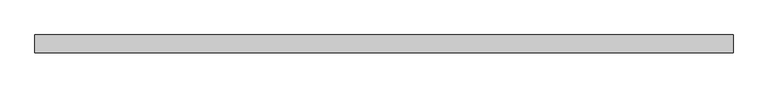
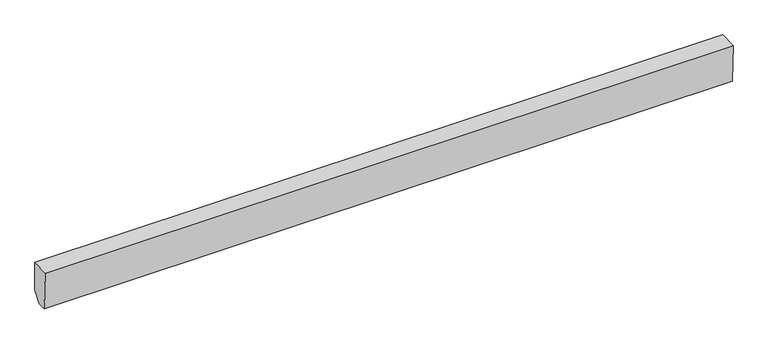
"""IFC4 building model written with IfcOpenShell, lengths in millimetres: proxy geometry, Generic Models 7:Generic Models 1:337419:Generic Models 1:337419 : Generic Models 7:Generic Models 1:337419:10 : Generic Models 7:Generic Models 1:337419:Generic Models 1:337419 : Generic Models 7:Generic Models 1:337419:301336."""

from ifc_helpers import new_model, si_unit, frame, origin, place, context, project, spatial, polyline, outline, extrude, source, transform, mapped, element, save


def generic_models_bc604923(model_context):
    return source(origin(), model_context, "Body", "SweptSolid", [
        extrude(outline(polyline([(-568260.1767006, 4122.14678), (-568318.6137092, 4119.7119047), (-568330.06354, 4394.5078449), (-568205.6913841, 4399.6900181), (-568205.6913841, 4192.8615123), (-568260.1767006, 4122.14678)])), frame((591306.0367242, 0.0, 0.0), z_axis=(1.0, 0.0, 0.0), x_axis=(0.0, 1.0, 0.0)), (0.0, 0.0, 1.0), 4876.8),
    ])


if __name__ == "__main__":
    model = new_model("IFC4")
    model_context = context("Model", 3, world=origin())
    ifc_project = project(units=[si_unit("LENGTHUNIT", "METRE", prefix="MILLI")], contexts=[model_context])
    site = spatial("IfcSite", under=ifc_project)
    building = spatial("IfcBuilding", under=site)
    placement = place(None, origin())
    generic_models_shape = generic_models_bc604923(model_context)
    element("IfcBuildingElementProxy", 1, Name="Generic Models 7:Generic Models 1:337419:Generic Models 1:337419 : Generic Models 7:Generic Models 1:337419:10 : Generic Models 7:Generic Models 1:337419:Generic Models 1:337419 : Generic Models 7:Generic Models 1:337419:301336", ObjectType="Generic Models 7:Generic Models 1:337419:Generic Models 1:337419 : Generic Models 7:Generic Models 1:337419:10 : Generic Models 7:Generic Models 1:337419:Generic Models 1:337419 : Generic Models 7:Generic Models 1:337419:301336", at=placement, inside=building, context=model_context, shape_type="MappedRepresentation", body=[
        mapped(generic_models_shape, transform((0.0, 0.0, 0.0), x_axis=(1.0, 0.0, 0.0), y_axis=(0.0, 1.0, 0.0), z_axis=(0.0, 0.0, 1.0))),
    ])
    save(model, "model.ifc")

# Revit data of these elements
# Type "Generic Models 7:Generic Models 1:337419:Generic Models 1:337419 : Generic Models 7:Generic Models 1:337419:10 : Generic Models 7:Generic Models 1:337419:Generic Models 1:337419 : Generic Models 7:Generic Models 1:337419:301336"
#   NameOverride = "Generic Models 7:Generic Models 1:337419:Generic Models 1:337419 : Generic Models 7:Generic Models 1:337419:301336"
#   ObjectTypeOverride = "Generic Models 1:337419 : Generic Models 7:Generic Models 1:337419"
#   Reference = "Generic Models 1"
#   Tag = "301336"
# Element 1 (IfcBuildingElementProxy, "Generic Models 7:Generic Models 1:337419:Generic Models 1:337419 : Generic Models 7:Generic Models 1:337419:10 : Generic Models 7:Generic Models 1:337419:Generic Models 1:337419 : Generic Models 7:Generic Models 1:337419:301336")
#   Materials on its faces: "LOW VOLUMN EXPANDABLE FOAM INSULATION"
# Materials
#   "LOW VOLUMN EXPANDABLE FOAM INSULATION": class "Unassigned", colour RGB 213 216 95, transparency 0, Cost = 0
